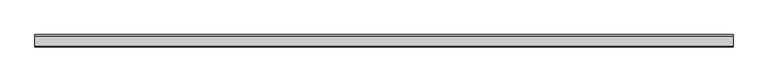
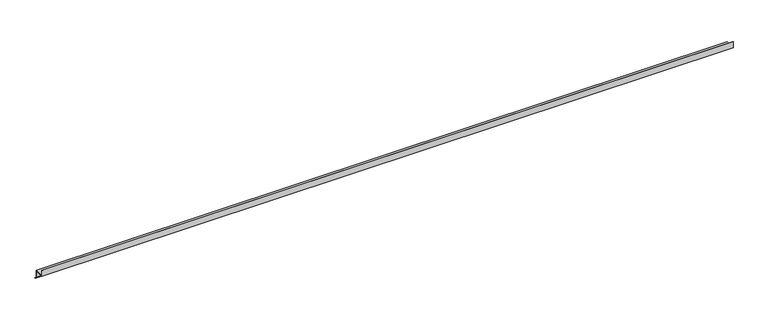
"""IFC4 building model written with IfcOpenShell, lengths in millimetres: proxy geometry, Generic Models 7:Generic Models 1:337419:Generic Models 1:337419 : Generic Models 7:Generic Models 1:337419:17 : Generic Models 7:Generic Models 1:337419:Generic Models 1:337419 : Generic Models 7:Generic Models 1:337419:301336."""

from ifc_helpers import new_model, si_unit, frame, origin, place, context, project, spatial, polyline, outline, extrude, source, transform, mapped, element, save


def generic_models_968e63c0(model_context):
    return source(origin(), model_context, "Body", "SweptSolid", [
        extrude(outline(polyline([(-536561.1796979, 8581.7240819), (-536561.1796979, 8627.084333), (-536558.4015729, 8627.084333), (-536558.4015729, 8584.5022069), (-536488.9484479, 8584.5022069), (-536488.9484479, 8533.7022069), (-536475.4780637, 8520.2318227), (-536477.4424947, 8518.2673917), (-536491.7265729, 8532.5514699), (-536491.7265729, 8581.7240819), (-536561.1796979, 8581.7240819)])), frame((591306.0367242, 0.0, 0.0), z_axis=(1.0, 0.0, 0.0), x_axis=(0.0, 1.0, 0.0)), (0.0, 0.0, 1.0), 4876.8),
    ])


if __name__ == "__main__":
    model = new_model("IFC4")
    model_context = context("Model", 3, world=origin())
    ifc_project = project(units=[si_unit("LENGTHUNIT", "METRE", prefix="MILLI")], contexts=[model_context])
    site = spatial("IfcSite", under=ifc_project)
    building = spatial("IfcBuilding", under=site)
    placement = place(None, origin())
    generic_models_shape = generic_models_968e63c0(model_context)
    element("IfcBuildingElementProxy", 1, Name="Generic Models 7:Generic Models 1:337419:Generic Models 1:337419 : Generic Models 7:Generic Models 1:337419:17 : Generic Models 7:Generic Models 1:337419:Generic Models 1:337419 : Generic Models 7:Generic Models 1:337419:301336", ObjectType="Generic Models 7:Generic Models 1:337419:Generic Models 1:337419 : Generic Models 7:Generic Models 1:337419:17 : Generic Models 7:Generic Models 1:337419:Generic Models 1:337419 : Generic Models 7:Generic Models 1:337419:301336", at=placement, inside=building, context=model_context, shape_type="MappedRepresentation", body=[
        mapped(generic_models_shape, transform((0.0, 0.0, 0.0), x_axis=(1.0, 0.0, 0.0), y_axis=(0.0, 1.0, 0.0), z_axis=(0.0, 0.0, 1.0))),
    ])
    save(model, "model.ifc")

# Revit data of these elements
# Type "Generic Models 7:Generic Models 1:337419:Generic Models 1:337419 : Generic Models 7:Generic Models 1:337419:17 : Generic Models 7:Generic Models 1:337419:Generic Models 1:337419 : Generic Models 7:Generic Models 1:337419:301336"
#   NameOverride = "Generic Models 7:Generic Models 1:337419:Generic Models 1:337419 : Generic Models 7:Generic Models 1:337419:301336"
#   ObjectTypeOverride = "Generic Models 1:337419 : Generic Models 7:Generic Models 1:337419"
#   Reference = "Generic Models 1"
#   Tag = "301336"
# Element 1 (IfcBuildingElementProxy, "Generic Models 7:Generic Models 1:337419:Generic Models 1:337419 : Generic Models 7:Generic Models 1:337419:17 : Generic Models 7:Generic Models 1:337419:Generic Models 1:337419 : Generic Models 7:Generic Models 1:337419:301336")
#   Materials on its faces: "BRAKE METAL FLASHING WITH BACK & END DAMS"
# Materials
#   "BRAKE METAL FLASHING WITH BACK & END DAMS": class "Unassigned", colour RGB 182 182 182, transparency 0, Cost = 0
